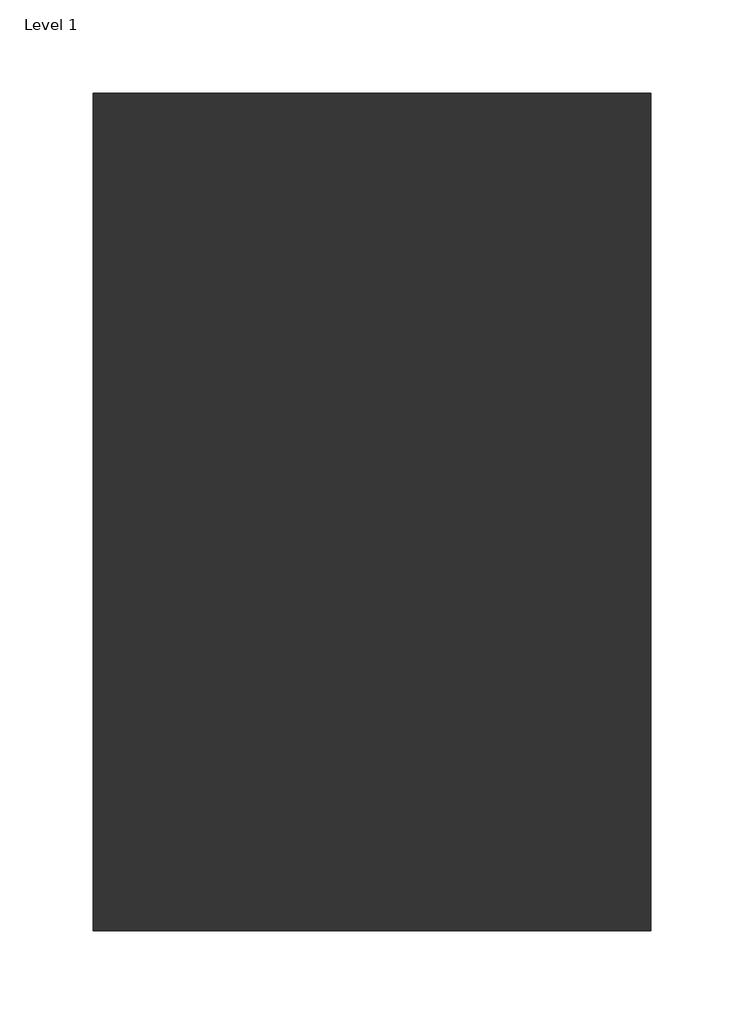
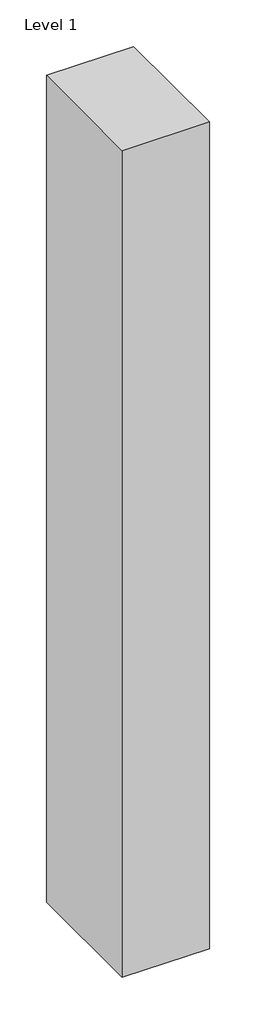
# One storey, part 1 of 2: 1 column.
"""IFC4 building model written with IfcOpenShell, lengths in millimetres."""

import ifcopenshell
import ifcopenshell.guid

model = None  # the IFC model being written
_history = None  # IfcOwnerHistory: only IFC2X3 demands one
_inside = {}  # id of a spatial element -> (the spatial element, [elements in it])
_under = {}  # id of a project, library or spatial element -> (it, [spatial elements below it])
_declared = {}  # id of a project -> (the project, [libraries it declares])
_typed = {}  # id of a type object -> (the type object, [elements of that type])
_made_of = {}  # id of a material, layer set ... -> (it, [elements and type objects made of it])


def new_model(schema):
    """Start an empty IFC model of exactly this schema.

    Asked for "IFC4X3", IfcOpenShell would pick the latest addendum, in which some entities
    have other attributes; the version numbers below select the first issue.
    IFC2X3 requires an IfcOwnerHistory on every rooted entity: one is made here for all.
    """
    global model, _history
    if schema == "IFC4X3":
        model = ifcopenshell.file(schema_version=(4, 3, 0, 0))
    else:
        model = ifcopenshell.file(schema=schema)
    _inside.clear()
    _under.clear()
    _declared.clear()
    _typed.clear()
    _made_of.clear()
    _history = None
    if model.schema == "IFC2X3":
        org = make("IfcOrganization", Name="unknown")
        user = make(
            "IfcPersonAndOrganization",
            ThePerson=make("IfcPerson", FamilyName="unknown"),
            TheOrganization=org,
        )
        app = make(
            "IfcApplication",
            ApplicationDeveloper=org,
            Version="unknown",
            ApplicationFullName="unknown",
            ApplicationIdentifier="unknown",
        )
        _history = make(
            "IfcOwnerHistory",
            OwningUser=user,
            OwningApplication=app,
            ChangeAction="ADDED",
            CreationDate=0,
        )
    return model


def make(cls, **values):
    """One entity of the class cls with the attributes given. An attribute that is None is left unset."""
    return model.create_entity(
        cls, **{name: value for name, value in values.items() if value is not None}
    )


def rooted(cls, **values):
    """An entity with a GlobalId (a new one), such as an element, a storey or a relation."""
    return make(cls, GlobalId=ifcopenshell.guid.new(), OwnerHistory=_history, **values)


def si_unit(unit_type, name, prefix=None):
    """IfcSIUnit, for example si_unit("LENGTHUNIT", "METRE", prefix="MILLI")."""
    return make("IfcSIUnit", UnitType=unit_type, Prefix=prefix, Name=name)


def assignment(units):
    """IfcUnitAssignment: the units of a project."""
    return None if units is None else make("IfcUnitAssignment", Units=units)


def point(xyz):
    """IfcCartesianPoint."""
    return None if xyz is None else make("IfcCartesianPoint", Coordinates=xyz)


def direction(xyz):
    """IfcDirection."""
    return None if xyz is None else make("IfcDirection", DirectionRatios=xyz)


def frame(location, z_axis=None, x_axis=None):
    """IfcAxis2Placement3D, a coordinate frame: its origin and axes. An axis left out is left unset."""
    return make(
        "IfcAxis2Placement3D",
        Location=point(location),
        Axis=direction(z_axis),
        RefDirection=direction(x_axis),
    )


def origin():
    """The frame at (0, 0, 0) with its axes left unset."""
    return frame((0.0, 0.0, 0.0))


def origin_with_axes():
    """The frame at (0, 0, 0) with the z axis (0, 0, 1) and the x axis (1, 0, 0) written out."""
    return frame((0.0, 0.0, 0.0), z_axis=(0.0, 0.0, 1.0), x_axis=(1.0, 0.0, 0.0))


def place(relative_to, where):
    """IfcLocalPlacement: puts the frame where relative to a parent placement (None: the world)."""
    return make(
        "IfcLocalPlacement", PlacementRelTo=relative_to, RelativePlacement=where
    )


def context(
    kind, dimensions, precision=None, world=None, true_north=None, identifier=None
):
    """IfcGeometricRepresentationContext, for example the 3D "Model" context."""
    return make(
        "IfcGeometricRepresentationContext",
        ContextIdentifier=identifier,
        ContextType=kind,
        CoordinateSpaceDimension=dimensions,
        Precision=precision,
        WorldCoordinateSystem=world,
        TrueNorth=true_north,
    )


def project(units=None, contexts=None):
    """IfcProject with its units and contexts."""
    return rooted(
        "IfcProject",
        Name="project",
        RepresentationContexts=contexts,
        UnitsInContext=assignment(units),
    )


def spatial(cls, under=None, at=None, **own):
    """A site, building, storey or space (cls), placed at a placement, below another one or the project."""
    s = rooted(cls, ObjectPlacement=at, **own)
    if under is not None:
        _under.setdefault(under.id(), (under, []))[1].append(s)
    return s


def polyline(points):
    """IfcPolyline through the points."""
    return make("IfcPolyline", Points=[point(p) for p in points])


def outline(outer, holes=None, kind="AREA"):
    """IfcArbitraryClosedProfileDef: a profile drawn as a closed curve; with holes, ...WithVoids."""
    if holes is None:
        return make("IfcArbitraryClosedProfileDef", ProfileType=kind, OuterCurve=outer)
    return make(
        "IfcArbitraryProfileDefWithVoids",
        ProfileType=kind,
        OuterCurve=outer,
        InnerCurves=holes,
    )


def extrude(swept, where, along, depth):
    """IfcExtrudedAreaSolid: the profile swept, set in the frame where, extruded along a direction by depth."""
    return make(
        "IfcExtrudedAreaSolid",
        SweptArea=swept,
        Position=where,
        ExtrudedDirection=direction(along),
        Depth=depth,
    )


def shape(context_of_items, identifier, shape_type, items):
    """IfcShapeRepresentation: the items that make up one representation, for example the "Body"."""
    return make(
        "IfcShapeRepresentation",
        ContextOfItems=context_of_items,
        RepresentationIdentifier=identifier,
        RepresentationType=shape_type,
        Items=items,
    )


def source(mapping_origin, context_of_items, identifier, shape_type, items):
    """IfcRepresentationMap: a shape defined once, which mapped items show again and again."""
    return make(
        "IfcRepresentationMap",
        MappingOrigin=mapping_origin,
        MappedRepresentation=shape(context_of_items, identifier, shape_type, items),
    )


def transform(
    local_origin,
    x_axis=None,
    y_axis=None,
    z_axis=None,
    scale=None,
    scale2=None,
    scale3=None,
    uniform=True,
):
    """IfcCartesianTransformationOperator3D, or its non-uniform kind. x_axis, y_axis, z_axis: its Axis1, 2, 3."""
    if uniform:
        return make(
            "IfcCartesianTransformationOperator3D",
            Axis1=direction(x_axis),
            Axis2=direction(y_axis),
            LocalOrigin=point(local_origin),
            Scale=scale,
            Axis3=direction(z_axis),
        )
    return make(
        "IfcCartesianTransformationOperator3DnonUniform",
        Axis1=direction(x_axis),
        Axis2=direction(y_axis),
        LocalOrigin=point(local_origin),
        Scale=scale,
        Axis3=direction(z_axis),
        Scale2=scale2,
        Scale3=scale3,
    )


def mapped(mapping_source, mapping_target):
    """IfcMappedItem: shows the shape of a source again, moved by a transform."""
    return make(
        "IfcMappedItem", MappingSource=mapping_source, MappingTarget=mapping_target
    )


def made_of(thing, what):
    """Note that an element or type object is made of a material, layer set ...; save() writes the relation."""
    if what is not None:
        _made_of.setdefault(what.id(), (what, []))[1].append(thing)
    return thing


def element(
    cls,
    number,
    at=None,
    inside=None,
    cuts=None,
    type_object=None,
    material=None,
    context=None,
    identifier="Body",
    shape_type=None,
    held_by="IfcProductDefinitionShape",
    body=None,
    shapes=None,
    **own,
):
    """One element of the class cls, such as IfcWall. Its Tag is "e" and its number.

    at: its placement. inside: the storey or other place that contains it. cuts: it is an
    opening in that element (IfcRelVoidsElement). A single representation is given by context,
    identifier, shape_type and body (its items); several are given by shapes. held_by: the class
    of the entity that holds the representations. save() writes the other relations.
    """
    e = rooted(cls, Tag="e%d" % number, ObjectPlacement=at, **own)
    if body is not None:
        shapes = [shape(context, identifier, shape_type, body)]
    if shapes is not None:
        e.Representation = make(held_by, Representations=shapes)
    if inside is not None:
        _inside.setdefault(inside.id(), (inside, []))[1].append(e)
    if cuts is not None:
        rooted(
            "IfcRelVoidsElement", RelatingBuildingElement=cuts, RelatedOpeningElement=e
        )
    if type_object is not None:
        _typed.setdefault(type_object.id(), (type_object, []))[1].append(e)
    return made_of(e, material)


def aggregate(whole, parts):
    """IfcRelAggregates: a whole, such as a stair, and the parts it consists of."""
    return rooted("IfcRelAggregates", RelatingObject=whole, RelatedObjects=parts)


def save(model, path):
    """Write the relations noted so far, then the file.

    IfcRelAggregates (storeys below a building ...), IfcRelContainedInSpatialStructure (elements
    in a storey), IfcRelDefinesByType, IfcRelAssociatesMaterial and IfcRelDeclares: one each for
    every whole, place, type object, material and project.
    """
    for whole, parts in _under.values():
        aggregate(whole, parts)
    for where, things in _inside.values():
        rooted(
            "IfcRelContainedInSpatialStructure",
            RelatedElements=things,
            RelatingStructure=where,
        )
    for kind, things in _typed.values():
        rooted("IfcRelDefinesByType", RelatedObjects=things, RelatingType=kind)
    for what, things in _made_of.values():
        rooted("IfcRelAssociatesMaterial", RelatedObjects=things, RelatingMaterial=what)
    for by, libraries in _declared.values():
        rooted("IfcRelDeclares", RelatingContext=by, RelatedDefinitions=libraries)
    model.write(path)


def concrete_rectangular_column_300_x_450mm_5cd98a27(model_context):
    return source(origin(), model_context, "Body", "SweptSolid", [
        extrude(outline(polyline([(150.0, 225.0), (150.0, -225.0), (-150.0, -225.0), (-150.0, 225.0), (150.0, 225.0)])), origin_with_axes(), (0.0, 0.0, 1.0), 3000.0),
    ])


model = new_model("IFC4")

# Units and contexts
model_context = context("Model", 3, world=origin())
ifc_project = project(units=[si_unit("LENGTHUNIT", "METRE", prefix="MILLI")], contexts=[model_context])

# Site, building, storey
site = spatial("IfcSite", under=ifc_project)
building = spatial("IfcBuilding", under=site)
storey = spatial("IfcBuildingStorey", under=building, Name="Level 1", Elevation=0.0)

# Column
placement = place(None, origin())
concrete_rectangular_column_300_x_450mm_shape = concrete_rectangular_column_300_x_450mm_5cd98a27(model_context)
element("IfcColumn", 1, ObjectType="Concrete-Rectangular-Column : 300 x 450mm", at=placement, inside=storey, context=model_context, shape_type="MappedRepresentation", body=[
    mapped(concrete_rectangular_column_300_x_450mm_shape, transform((-8094.162791, 1629.0953602, 0.0), x_axis=(1.0, 0.0, 0.0), y_axis=(0.0, 1.0, 0.0), z_axis=(0.0, 0.0, 1.0))),
])

save(model, "model.ifc")

# Revit data of these elements
# Project information
#   Project Issue Date = "Issue Date"
#   Project Status = "Project Status"
#   Client Name = "Owner"
#   Project Address = "Enter address here"
#   Project Name = "Project Name"
#   Project Number = "Project Number"
# Type "Concrete-Rectangular-Column : 300 x 450mm"
#   b = 300 mm
#   h = 450 mm
#   Structural Material [instance default] = Concrete, Cast-in-Place gray
# Element 1 (IfcColumn, "Concrete-Rectangular-Column : 300 x 450mm")
#   Mark = "C1"
#   Phase Created = New Construction
#   Materials on its faces: "Concrete, Cast-in-Place gray"
# Materials
#   "Concrete, Cast-in-Place gray": class "Concrete", colour RGB 192 192 192, transparency 0, Description = "Cast-in-place concrete", Cost = 0
